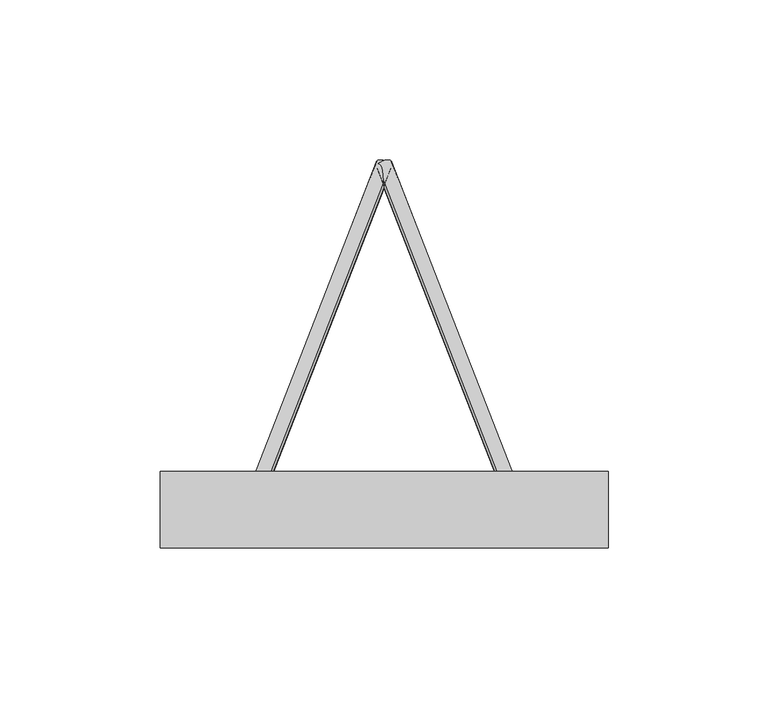
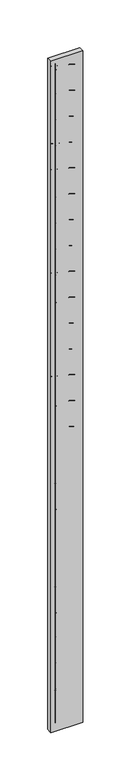
"""IFC4 building model written with IfcOpenShell, lengths in millimetres: proxy geometry, Vigota 1 (Pano 3) (Mf = 803)."""

from ifc_helpers import new_model, si_unit, point, frame, frame_2d, origin, origin_with_axes, origin_2d, place, context, project, spatial, polyline, circle_curve, trimmed, segment, composite_curve, outline, extrude, source, transform, mapped, element, save


def structural_framing_3061a772(model_context):
    return source(origin(), model_context, "Body", "SweptSolid", [
        extrude(outline(polyline([(-70.0, 12.0), (70.0, 12.0), (70.0, -12.0), (-70.0, -12.0), (-70.0, 12.0)])), origin_with_axes(), (0.0, 0.0, 1.0), 3115.00107),
        extrude(outline(composite_curve([segment(trimmed(circle_curve(origin_2d(), 2.5), [point((2.5, 0.0))], [point((-2.5, 0.0))], False, "CARTESIAN"), True, "CONTINUOUS"), segment(trimmed(circle_curve(origin_2d(), 2.5), [point((-2.5, 0.0))], [point((2.5, 0.0))], False, "CARTESIAN"), True, "CONTINUOUS")], self_intersect=False)), frame((0.0, 108.0, 1317.500535), z_axis=(0.3218603428886276, -0.8276408817707567, 0.4598004898837537), x_axis=(0.8192319205108605, -3.936835275445103e-11, -0.5734623443750141)), (0.0, 0.0, 1.0), 130.491379),
        extrude(outline(composite_curve([segment(trimmed(circle_curve(origin_2d(), 2.5), [point((2.5, 0.0))], [point((-2.5, 0.0))], False, "CARTESIAN"), True, "CONTINUOUS"), segment(trimmed(circle_curve(origin_2d(), 2.5), [point((-2.5, 0.0))], [point((2.5, 0.0))], False, "CARTESIAN"), True, "CONTINUOUS")], self_intersect=False)), frame((42.0, 0.0, 1377.500535), z_axis=(-0.3218603428886276, 0.8276408817707567, 0.4598004898837537), x_axis=(0.8192319205108605, -3.936835275445103e-11, 0.5734623443750141)), (0.0, 0.0, 1.0), 130.491379),
        extrude(outline(composite_curve([segment(trimmed(circle_curve(origin_2d(), 2.5), [point((2.5, 0.0))], [point((-2.5, 0.0))], False, "CARTESIAN"), True, "CONTINUOUS"), segment(trimmed(circle_curve(origin_2d(), 2.5), [point((-2.5, 0.0))], [point((2.5, 0.0))], False, "CARTESIAN"), True, "CONTINUOUS")], self_intersect=False)), frame((0.0, 108.0, 1437.500535), z_axis=(0.3218603428886276, -0.8276408817707567, 0.4598004898837537), x_axis=(0.8192319205108605, -3.936835275445103e-11, -0.5734623443750141)), (0.0, 0.0, 1.0), 130.491379),
        extrude(outline(composite_curve([segment(trimmed(circle_curve(origin_2d(), 2.5), [point((2.5, 0.0))], [point((-2.5, 0.0))], False, "CARTESIAN"), True, "CONTINUOUS"), segment(trimmed(circle_curve(origin_2d(), 2.5), [point((-2.5, 0.0))], [point((2.5, 0.0))], False, "CARTESIAN"), True, "CONTINUOUS")], self_intersect=False)), frame((42.0, 0.0, 1497.500535), z_axis=(-0.3218603428886276, 0.8276408817707567, 0.4598004898837537), x_axis=(0.8192319205108605, -3.936835275445103e-11, 0.5734623443750141)), (0.0, 0.0, 1.0), 130.491379),
        extrude(outline(composite_curve([segment(trimmed(circle_curve(origin_2d(), 2.5), [point((2.5, 0.0))], [point((-2.5, 0.0))], False, "CARTESIAN"), True, "CONTINUOUS"), segment(trimmed(circle_curve(origin_2d(), 2.5), [point((-2.5, 0.0))], [point((2.5, 0.0))], False, "CARTESIAN"), True, "CONTINUOUS")], self_intersect=False)), frame((0.0, 108.0, 1557.500535), z_axis=(0.3218603428886276, -0.8276408817707567, 0.4598004898837537), x_axis=(0.8192319205108605, -3.936835275445103e-11, -0.5734623443750141)), (0.0, 0.0, 1.0), 130.491379),
        extrude(outline(composite_curve([segment(trimmed(circle_curve(origin_2d(), 2.5), [point((2.5, 0.0))], [point((-2.5, 0.0))], False, "CARTESIAN"), True, "CONTINUOUS"), segment(trimmed(circle_curve(origin_2d(), 2.5), [point((-2.5, 0.0))], [point((2.5, 0.0))], False, "CARTESIAN"), True, "CONTINUOUS")], self_intersect=False)), frame((42.0, 0.0, 1617.500535), z_axis=(-0.3218603428886276, 0.8276408817707567, 0.4598004898837537), x_axis=(0.8192319205108605, -3.936835275445103e-11, 0.5734623443750141)), (0.0, 0.0, 1.0), 130.491379),
        extrude(outline(composite_curve([segment(trimmed(circle_curve(origin_2d(), 2.5), [point((2.5, 0.0))], [point((-2.5, 0.0))], False, "CARTESIAN"), True, "CONTINUOUS"), segment(trimmed(circle_curve(origin_2d(), 2.5), [point((-2.5, 0.0))], [point((2.5, 0.0))], False, "CARTESIAN"), True, "CONTINUOUS")], self_intersect=False)), frame((0.0, 108.0, 1677.500535), z_axis=(0.3218603428886276, -0.8276408817707567, 0.4598004898837537), x_axis=(0.8192319205108605, -3.936835275445103e-11, -0.5734623443750141)), (0.0, 0.0, 1.0), 130.491379),
        extrude(outline(composite_curve([segment(trimmed(circle_curve(origin_2d(), 2.5), [point((2.5, 0.0))], [point((-2.5, 0.0))], False, "CARTESIAN"), True, "CONTINUOUS"), segment(trimmed(circle_curve(origin_2d(), 2.5), [point((-2.5, 0.0))], [point((2.5, 0.0))], False, "CARTESIAN"), True, "CONTINUOUS")], self_intersect=False)), frame((42.0, 0.0, 1737.500535), z_axis=(-0.3218603428886276, 0.8276408817707567, 0.4598004898837537), x_axis=(0.8192319205108605, -3.936835275445103e-11, 0.5734623443750141)), (0.0, 0.0, 1.0), 130.491379),
        extrude(outline(composite_curve([segment(trimmed(circle_curve(origin_2d(), 2.5), [point((2.5, 0.0))], [point((-2.5, 0.0))], False, "CARTESIAN"), True, "CONTINUOUS"), segment(trimmed(circle_curve(origin_2d(), 2.5), [point((-2.5, 0.0))], [point((2.5, 0.0))], False, "CARTESIAN"), True, "CONTINUOUS")], self_intersect=False)), frame((0.0, 108.0, 1797.500535), z_axis=(0.3218603428886276, -0.8276408817707567, 0.4598004898837537), x_axis=(0.8192319205108605, -3.936835275445103e-11, -0.5734623443750141)), (0.0, 0.0, 1.0), 130.491379),
        extrude(outline(composite_curve([segment(trimmed(circle_curve(origin_2d(), 2.5), [point((2.5, 0.0))], [point((-2.5, 0.0))], False, "CARTESIAN"), True, "CONTINUOUS"), segment(trimmed(circle_curve(origin_2d(), 2.5), [point((-2.5, 0.0))], [point((2.5, 0.0))], False, "CARTESIAN"), True, "CONTINUOUS")], self_intersect=False)), frame((42.0, 0.0, 1857.500535), z_axis=(-0.3218603428886276, 0.8276408817707567, 0.4598004898837537), x_axis=(0.8192319205108605, -3.936835275445103e-11, 0.5734623443750141)), (0.0, 0.0, 1.0), 130.491379),
        extrude(outline(composite_curve([segment(trimmed(circle_curve(origin_2d(), 2.5), [point((2.5, 0.0))], [point((-2.5, 0.0))], False, "CARTESIAN"), True, "CONTINUOUS"), segment(trimmed(circle_curve(origin_2d(), 2.5), [point((-2.5, 0.0))], [point((2.5, 0.0))], False, "CARTESIAN"), True, "CONTINUOUS")], self_intersect=False)), frame((0.0, 108.0, 1917.500535), z_axis=(0.3218603428886276, -0.8276408817707567, 0.4598004898837537), x_axis=(0.8192319205108605, -3.936835275445103e-11, -0.5734623443750141)), (0.0, 0.0, 1.0), 130.491379),
        extrude(outline(composite_curve([segment(trimmed(circle_curve(origin_2d(), 2.5), [point((2.5, 0.0))], [point((-2.5, 0.0))], False, "CARTESIAN"), True, "CONTINUOUS"), segment(trimmed(circle_curve(origin_2d(), 2.5), [point((-2.5, 0.0))], [point((2.5, 0.0))], False, "CARTESIAN"), True, "CONTINUOUS")], self_intersect=False)), frame((42.0, 0.0, 1977.500535), z_axis=(-0.3218603428886276, 0.8276408817707567, 0.4598004898837537), x_axis=(0.8192319205108605, -3.936835275445103e-11, 0.5734623443750141)), (0.0, 0.0, 1.0), 130.491379),
        extrude(outline(composite_curve([segment(trimmed(circle_curve(origin_2d(), 2.5), [point((2.5, 0.0))], [point((-2.5, 0.0))], False, "CARTESIAN"), True, "CONTINUOUS"), segment(trimmed(circle_curve(origin_2d(), 2.5), [point((-2.5, 0.0))], [point((2.5, 0.0))], False, "CARTESIAN"), True, "CONTINUOUS")], self_intersect=False)), frame((0.0, 108.0, 2037.500535), z_axis=(0.3218603428886276, -0.8276408817707567, 0.4598004898837537), x_axis=(0.8192319205108605, -3.936835275445103e-11, -0.5734623443750141)), (0.0, 0.0, 1.0), 130.491379),
        extrude(outline(composite_curve([segment(trimmed(circle_curve(origin_2d(), 2.5), [point((2.5, 0.0))], [point((-2.5, 0.0))], False, "CARTESIAN"), True, "CONTINUOUS"), segment(trimmed(circle_curve(origin_2d(), 2.5), [point((-2.5, 0.0))], [point((2.5, 0.0))], False, "CARTESIAN"), True, "CONTINUOUS")], self_intersect=False)), frame((42.0, 0.0, 2097.500535), z_axis=(-0.3218603428886276, 0.8276408817707567, 0.4598004898837537), x_axis=(0.8192319205108605, -3.936835275445103e-11, 0.5734623443750141)), (0.0, 0.0, 1.0), 130.491379),
        extrude(outline(composite_curve([segment(trimmed(circle_curve(origin_2d(), 2.5), [point((2.5, 0.0))], [point((-2.5, 0.0))], False, "CARTESIAN"), True, "CONTINUOUS"), segment(trimmed(circle_curve(origin_2d(), 2.5), [point((-2.5, 0.0))], [point((2.5, 0.0))], False, "CARTESIAN"), True, "CONTINUOUS")], self_intersect=False)), frame((0.0, 108.0, 2157.500535), z_axis=(0.3218603428886276, -0.8276408817707567, 0.4598004898837537), x_axis=(0.8192319205108605, -3.936835275445103e-11, -0.5734623443750141)), (0.0, 0.0, 1.0), 130.491379),
        extrude(outline(composite_curve([segment(trimmed(circle_curve(origin_2d(), 2.5), [point((2.5, 0.0))], [point((-2.5, 0.0))], False, "CARTESIAN"), True, "CONTINUOUS"), segment(trimmed(circle_curve(origin_2d(), 2.5), [point((-2.5, 0.0))], [point((2.5, 0.0))], False, "CARTESIAN"), True, "CONTINUOUS")], self_intersect=False)), frame((42.0, 0.0, 2217.500535), z_axis=(-0.3218603428886276, 0.8276408817707567, 0.4598004898837537), x_axis=(0.8192319205108605, -3.936835275445103e-11, 0.5734623443750141)), (0.0, 0.0, 1.0), 130.491379),
        extrude(outline(composite_curve([segment(trimmed(circle_curve(origin_2d(), 2.5), [point((2.5, 0.0))], [point((-2.5, 0.0))], False, "CARTESIAN"), True, "CONTINUOUS"), segment(trimmed(circle_curve(origin_2d(), 2.5), [point((-2.5, 0.0))], [point((2.5, 0.0))], False, "CARTESIAN"), True, "CONTINUOUS")], self_intersect=False)), frame((0.0, 108.0, 2277.500535), z_axis=(0.3218603428886276, -0.8276408817707567, 0.4598004898837537), x_axis=(0.8192319205108605, -3.936835275445103e-11, -0.5734623443750141)), (0.0, 0.0, 1.0), 130.491379),
        extrude(outline(composite_curve([segment(trimmed(circle_curve(origin_2d(), 2.5), [point((2.5, 0.0))], [point((-2.5, 0.0))], False, "CARTESIAN"), True, "CONTINUOUS"), segment(trimmed(circle_curve(origin_2d(), 2.5), [point((-2.5, 0.0))], [point((2.5, 0.0))], False, "CARTESIAN"), True, "CONTINUOUS")], self_intersect=False)), frame((42.0, 0.0, 2337.500535), z_axis=(-0.3218603428886276, 0.8276408817707567, 0.4598004898837537), x_axis=(0.8192319205108605, -3.936835275445103e-11, 0.5734623443750141)), (0.0, 0.0, 1.0), 130.491379),
        extrude(outline(composite_curve([segment(trimmed(circle_curve(origin_2d(), 2.5), [point((2.5, 0.0))], [point((-2.5, 0.0))], False, "CARTESIAN"), True, "CONTINUOUS"), segment(trimmed(circle_curve(origin_2d(), 2.5), [point((-2.5, 0.0))], [point((2.5, 0.0))], False, "CARTESIAN"), True, "CONTINUOUS")], self_intersect=False)), frame((0.0, 108.0, 2397.500535), z_axis=(0.3218603428886276, -0.8276408817707567, 0.4598004898837537), x_axis=(0.8192319205108605, -3.936835275445103e-11, -0.5734623443750141)), (0.0, 0.0, 1.0), 130.491379),
        extrude(outline(composite_curve([segment(trimmed(circle_curve(origin_2d(), 2.5), [point((2.5, 0.0))], [point((-2.5, 0.0))], False, "CARTESIAN"), True, "CONTINUOUS"), segment(trimmed(circle_curve(origin_2d(), 2.5), [point((-2.5, 0.0))], [point((2.5, 0.0))], False, "CARTESIAN"), True, "CONTINUOUS")], self_intersect=False)), frame((42.0, 0.0, 2457.500535), z_axis=(-0.3218603428886276, 0.8276408817707567, 0.4598004898837537), x_axis=(0.8192319205108605, -3.936835275445103e-11, 0.5734623443750141)), (0.0, 0.0, 1.0), 130.491379),
        extrude(outline(composite_curve([segment(trimmed(circle_curve(origin_2d(), 2.5), [point((2.5, 0.0))], [point((-2.5, 0.0))], False, "CARTESIAN"), True, "CONTINUOUS"), segment(trimmed(circle_curve(origin_2d(), 2.5), [point((-2.5, 0.0))], [point((2.5, 0.0))], False, "CARTESIAN"), True, "CONTINUOUS")], self_intersect=False)), frame((0.0, 108.0, 2517.500535), z_axis=(0.3218603428886276, -0.8276408817707567, 0.4598004898837537), x_axis=(0.8192319205108605, -3.936835275445103e-11, -0.5734623443750141)), (0.0, 0.0, 1.0), 130.491379),
        extrude(outline(composite_curve([segment(trimmed(circle_curve(origin_2d(), 2.5), [point((2.5, 0.0))], [point((-2.5, 0.0))], False, "CARTESIAN"), True, "CONTINUOUS"), segment(trimmed(circle_curve(origin_2d(), 2.5), [point((-2.5, 0.0))], [point((2.5, 0.0))], False, "CARTESIAN"), True, "CONTINUOUS")], self_intersect=False)), frame((42.0, 0.0, 2577.500535), z_axis=(-0.3218603428886276, 0.8276408817707567, 0.4598004898837537), x_axis=(0.8192319205108605, -3.936835275445103e-11, 0.5734623443750141)), (0.0, 0.0, 1.0), 130.491379),
        extrude(outline(composite_curve([segment(trimmed(circle_curve(origin_2d(), 2.5), [point((2.5, 0.0))], [point((-2.5, 0.0))], False, "CARTESIAN"), True, "CONTINUOUS"), segment(trimmed(circle_curve(origin_2d(), 2.5), [point((-2.5, 0.0))], [point((2.5, 0.0))], False, "CARTESIAN"), True, "CONTINUOUS")], self_intersect=False)), frame((0.0, 108.0, 2637.500535), z_axis=(0.3218603428886276, -0.8276408817707567, 0.4598004898837537), x_axis=(0.8192319205108605, -3.936835275445103e-11, -0.5734623443750141)), (0.0, 0.0, 1.0), 130.491379),
        extrude(outline(composite_curve([segment(trimmed(circle_curve(origin_2d(), 2.5), [point((2.5, 0.0))], [point((-2.5, 0.0))], False, "CARTESIAN"), True, "CONTINUOUS"), segment(trimmed(circle_curve(origin_2d(), 2.5), [point((-2.5, 0.0))], [point((2.5, 0.0))], False, "CARTESIAN"), True, "CONTINUOUS")], self_intersect=False)), frame((42.0, 0.0, 2697.500535), z_axis=(-0.3218603428886276, 0.8276408817707567, 0.4598004898837537), x_axis=(0.8192319205108605, -3.936835275445103e-11, 0.5734623443750141)), (0.0, 0.0, 1.0), 130.491379),
        extrude(outline(composite_curve([segment(trimmed(circle_curve(origin_2d(), 2.5), [point((2.5, 0.0))], [point((-2.5, 0.0))], False, "CARTESIAN"), True, "CONTINUOUS"), segment(trimmed(circle_curve(origin_2d(), 2.5), [point((-2.5, 0.0))], [point((2.5, 0.0))], False, "CARTESIAN"), True, "CONTINUOUS")], self_intersect=False)), frame((0.0, 108.0, 2757.500535), z_axis=(0.3218603428886276, -0.8276408817707567, 0.4598004898837537), x_axis=(0.8192319205108605, -3.936835275445103e-11, -0.5734623443750141)), (0.0, 0.0, 1.0), 130.491379),
        extrude(outline(composite_curve([segment(trimmed(circle_curve(origin_2d(), 2.5), [point((2.5, 0.0))], [point((-2.5, 0.0))], False, "CARTESIAN"), True, "CONTINUOUS"), segment(trimmed(circle_curve(origin_2d(), 2.5), [point((-2.5, 0.0))], [point((2.5, 0.0))], False, "CARTESIAN"), True, "CONTINUOUS")], self_intersect=False)), frame((42.0, 0.0, 2817.500535), z_axis=(-0.3218603428886276, 0.8276408817707567, 0.4598004898837537), x_axis=(0.8192319205108605, -3.936835275445103e-11, 0.5734623443750141)), (0.0, 0.0, 1.0), 130.491379),
        extrude(outline(composite_curve([segment(trimmed(circle_curve(origin_2d(), 2.5), [point((2.5, 0.0))], [point((-2.5, 0.0))], False, "CARTESIAN"), True, "CONTINUOUS"), segment(trimmed(circle_curve(origin_2d(), 2.5), [point((-2.5, 0.0))], [point((2.5, 0.0))], False, "CARTESIAN"), True, "CONTINUOUS")], self_intersect=False)), frame((0.0, 108.0, 2877.500535), z_axis=(0.3218603428886276, -0.8276408817707567, 0.4598004898837537), x_axis=(0.8192319205108605, -3.936835275445103e-11, -0.5734623443750141)), (0.0, 0.0, 1.0), 130.491379),
        extrude(outline(composite_curve([segment(trimmed(circle_curve(origin_2d(), 2.5), [point((2.5, 0.0))], [point((-2.5, 0.0))], False, "CARTESIAN"), True, "CONTINUOUS"), segment(trimmed(circle_curve(origin_2d(), 2.5), [point((-2.5, 0.0))], [point((2.5, 0.0))], False, "CARTESIAN"), True, "CONTINUOUS")], self_intersect=False)), frame((42.0, 0.0, 2937.500535), z_axis=(-0.3218603428886276, 0.8276408817707567, 0.4598004898837537), x_axis=(0.8192319205108605, -3.936835275445103e-11, 0.5734623443750141)), (0.0, 0.0, 1.0), 130.491379),
        extrude(outline(composite_curve([segment(trimmed(circle_curve(origin_2d(), 2.5), [point((2.5, 0.0))], [point((-2.5, 0.0))], False, "CARTESIAN"), True, "CONTINUOUS"), segment(trimmed(circle_curve(origin_2d(), 2.5), [point((-2.5, 0.0))], [point((2.5, 0.0))], False, "CARTESIAN"), True, "CONTINUOUS")], self_intersect=False)), frame((0.0, 108.0, 2997.500535), z_axis=(0.3218603428886276, -0.8276408817707567, 0.4598004898837537), x_axis=(0.8192319205108605, -3.936835275445103e-11, -0.5734623443750141)), (0.0, 0.0, 1.0), 130.491379),
        extrude(outline(composite_curve([segment(trimmed(circle_curve(frame_2d((-42.0, 0.0)), 2.5), [point((-39.5, 0.0))], [point((-44.5, 0.0))], False, "CARTESIAN"), True, "CONTINUOUS"), segment(trimmed(circle_curve(frame_2d((-42.0, 0.0)), 2.5), [point((-44.5, 0.0))], [point((-39.5, 0.0))], False, "CARTESIAN"), True, "CONTINUOUS")], self_intersect=False)), frame((0.0, 0.0, 28.0), z_axis=(0.0, 0.0, 1.0), x_axis=(1.0, 0.0, 0.0)), (0.0, 0.0, 1.0), 3059.00107),
        extrude(outline(composite_curve([segment(trimmed(circle_curve(origin_2d(), 2.5), [point((2.5, 0.0))], [point((-2.5, 0.0))], False, "CARTESIAN"), True, "CONTINUOUS"), segment(trimmed(circle_curve(origin_2d(), 2.5), [point((-2.5, 0.0))], [point((2.5, 0.0))], False, "CARTESIAN"), True, "CONTINUOUS")], self_intersect=False)), frame((-42.0, 0.0, 57.500535), z_axis=(0.3218603428886276, 0.8276408817707567, 0.4598004898837537), x_axis=(0.8192319205108605, 3.936835275445103e-11, -0.5734623443750141)), (0.0, 0.0, 1.0), 130.491379),
        extrude(outline(composite_curve([segment(trimmed(circle_curve(origin_2d(), 2.5), [point((2.5, 0.0))], [point((-2.5, 0.0))], False, "CARTESIAN"), True, "CONTINUOUS"), segment(trimmed(circle_curve(origin_2d(), 2.5), [point((-2.5, 0.0))], [point((2.5, 0.0))], False, "CARTESIAN"), True, "CONTINUOUS")], self_intersect=False)), frame((0.0, 108.0, 117.500535), z_axis=(-0.3218603428886276, -0.8276408817707567, 0.4598004898837537), x_axis=(0.8192319205108605, 3.936835275445103e-11, 0.5734623443750141)), (0.0, 0.0, 1.0), 130.491379),
        extrude(outline(composite_curve([segment(trimmed(circle_curve(origin_2d(), 2.5), [point((2.5, 0.0))], [point((-2.5, 0.0))], False, "CARTESIAN"), True, "CONTINUOUS"), segment(trimmed(circle_curve(origin_2d(), 2.5), [point((-2.5, 0.0))], [point((2.5, 0.0))], False, "CARTESIAN"), True, "CONTINUOUS")], self_intersect=False)), frame((-42.0, 0.0, 177.500535), z_axis=(0.3218603428886276, 0.8276408817707567, 0.4598004898837537), x_axis=(0.8192319205108605, 3.936835275445103e-11, -0.5734623443750141)), (0.0, 0.0, 1.0), 130.491379),
        extrude(outline(composite_curve([segment(trimmed(circle_curve(origin_2d(), 2.5), [point((2.5, 0.0))], [point((-2.5, 0.0))], False, "CARTESIAN"), True, "CONTINUOUS"), segment(trimmed(circle_curve(origin_2d(), 2.5), [point((-2.5, 0.0))], [point((2.5, 0.0))], False, "CARTESIAN"), True, "CONTINUOUS")], self_intersect=False)), frame((0.0, 108.0, 237.500535), z_axis=(-0.3218603428886276, -0.8276408817707567, 0.4598004898837537), x_axis=(0.8192319205108605, 3.936835275445103e-11, 0.5734623443750141)), (0.0, 0.0, 1.0), 130.491379),
        extrude(outline(composite_curve([segment(trimmed(circle_curve(origin_2d(), 2.5), [point((2.5, 0.0))], [point((-2.5, 0.0))], False, "CARTESIAN"), True, "CONTINUOUS"), segment(trimmed(circle_curve(origin_2d(), 2.5), [point((-2.5, 0.0))], [point((2.5, 0.0))], False, "CARTESIAN"), True, "CONTINUOUS")], self_intersect=False)), frame((-42.0, 0.0, 297.500535), z_axis=(0.3218603428886276, 0.8276408817707567, 0.4598004898837537), x_axis=(0.8192319205108605, 3.936835275445103e-11, -0.5734623443750141)), (0.0, 0.0, 1.0), 130.491379),
        extrude(outline(composite_curve([segment(trimmed(circle_curve(origin_2d(), 2.5), [point((2.5, 0.0))], [point((-2.5, 0.0))], False, "CARTESIAN"), True, "CONTINUOUS"), segment(trimmed(circle_curve(origin_2d(), 2.5), [point((-2.5, 0.0))], [point((2.5, 0.0))], False, "CARTESIAN"), True, "CONTINUOUS")], self_intersect=False)), frame((0.0, 108.0, 357.500535), z_axis=(-0.3218603428886276, -0.8276408817707567, 0.4598004898837537), x_axis=(0.8192319205108605, 3.936835275445103e-11, 0.5734623443750141)), (0.0, 0.0, 1.0), 130.491379),
        extrude(outline(composite_curve([segment(trimmed(circle_curve(origin_2d(), 2.5), [point((2.5, 0.0))], [point((-2.5, 0.0))], False, "CARTESIAN"), True, "CONTINUOUS"), segment(trimmed(circle_curve(origin_2d(), 2.5), [point((-2.5, 0.0))], [point((2.5, 0.0))], False, "CARTESIAN"), True, "CONTINUOUS")], self_intersect=False)), frame((-42.0, 0.0, 417.500535), z_axis=(0.3218603428886276, 0.8276408817707567, 0.4598004898837537), x_axis=(0.8192319205108605, 3.936835275445103e-11, -0.5734623443750141)), (0.0, 0.0, 1.0), 130.491379),
        extrude(outline(composite_curve([segment(trimmed(circle_curve(origin_2d(), 2.5), [point((2.5, 0.0))], [point((-2.5, 0.0))], False, "CARTESIAN"), True, "CONTINUOUS"), segment(trimmed(circle_curve(origin_2d(), 2.5), [point((-2.5, 0.0))], [point((2.5, 0.0))], False, "CARTESIAN"), True, "CONTINUOUS")], self_intersect=False)), frame((0.0, 108.0, 477.500535), z_axis=(-0.3218603428886276, -0.8276408817707567, 0.4598004898837537), x_axis=(0.8192319205108605, 3.936835275445103e-11, 0.5734623443750141)), (0.0, 0.0, 1.0), 130.491379),
        extrude(outline(composite_curve([segment(trimmed(circle_curve(origin_2d(), 2.5), [point((2.5, 0.0))], [point((-2.5, 0.0))], False, "CARTESIAN"), True, "CONTINUOUS"), segment(trimmed(circle_curve(origin_2d(), 2.5), [point((-2.5, 0.0))], [point((2.5, 0.0))], False, "CARTESIAN"), True, "CONTINUOUS")], self_intersect=False)), frame((-42.0, 0.0, 537.500535), z_axis=(0.3218603428886276, 0.8276408817707567, 0.4598004898837537), x_axis=(0.8192319205108605, 3.936835275445103e-11, -0.5734623443750141)), (0.0, 0.0, 1.0), 130.491379),
        extrude(outline(composite_curve([segment(trimmed(circle_curve(origin_2d(), 2.5), [point((2.5, 0.0))], [point((-2.5, 0.0))], False, "CARTESIAN"), True, "CONTINUOUS"), segment(trimmed(circle_curve(origin_2d(), 2.5), [point((-2.5, 0.0))], [point((2.5, 0.0))], False, "CARTESIAN"), True, "CONTINUOUS")], self_intersect=False)), frame((0.0, 108.0, 597.500535), z_axis=(-0.3218603428886276, -0.8276408817707567, 0.4598004898837537), x_axis=(0.8192319205108605, 3.936835275445103e-11, 0.5734623443750141)), (0.0, 0.0, 1.0), 130.491379),
        extrude(outline(composite_curve([segment(trimmed(circle_curve(origin_2d(), 2.5), [point((2.5, 0.0))], [point((-2.5, 0.0))], False, "CARTESIAN"), True, "CONTINUOUS"), segment(trimmed(circle_curve(origin_2d(), 2.5), [point((-2.5, 0.0))], [point((2.5, 0.0))], False, "CARTESIAN"), True, "CONTINUOUS")], self_intersect=False)), frame((-42.0, 0.0, 657.500535), z_axis=(0.3218603428886276, 0.8276408817707567, 0.4598004898837537), x_axis=(0.8192319205108605, 3.936835275445103e-11, -0.5734623443750141)), (0.0, 0.0, 1.0), 130.491379),
        extrude(outline(composite_curve([segment(trimmed(circle_curve(origin_2d(), 2.5), [point((2.5, 0.0))], [point((-2.5, 0.0))], False, "CARTESIAN"), True, "CONTINUOUS"), segment(trimmed(circle_curve(origin_2d(), 2.5), [point((-2.5, 0.0))], [point((2.5, 0.0))], False, "CARTESIAN"), True, "CONTINUOUS")], self_intersect=False)), frame((0.0, 108.0, 717.500535), z_axis=(-0.3218603428886276, -0.8276408817707567, 0.4598004898837537), x_axis=(0.8192319205108605, 3.936835275445103e-11, 0.5734623443750141)), (0.0, 0.0, 1.0), 130.491379),
        extrude(outline(composite_curve([segment(trimmed(circle_curve(origin_2d(), 2.5), [point((2.5, 0.0))], [point((-2.5, 0.0))], False, "CARTESIAN"), True, "CONTINUOUS"), segment(trimmed(circle_curve(origin_2d(), 2.5), [point((-2.5, 0.0))], [point((2.5, 0.0))], False, "CARTESIAN"), True, "CONTINUOUS")], self_intersect=False)), frame((-42.0, 0.0, 777.500535), z_axis=(0.3218603428886276, 0.8276408817707567, 0.4598004898837537), x_axis=(0.8192319205108605, 3.936835275445103e-11, -0.5734623443750141)), (0.0, 0.0, 1.0), 130.491379),
        extrude(outline(composite_curve([segment(trimmed(circle_curve(origin_2d(), 2.5), [point((2.5, 0.0))], [point((-2.5, 0.0))], False, "CARTESIAN"), True, "CONTINUOUS"), segment(trimmed(circle_curve(origin_2d(), 2.5), [point((-2.5, 0.0))], [point((2.5, 0.0))], False, "CARTESIAN"), True, "CONTINUOUS")], self_intersect=False)), frame((0.0, 108.0, 837.500535), z_axis=(-0.3218603428886276, -0.8276408817707567, 0.4598004898837537), x_axis=(0.8192319205108605, 3.936835275445103e-11, 0.5734623443750141)), (0.0, 0.0, 1.0), 130.491379),
        extrude(outline(composite_curve([segment(trimmed(circle_curve(origin_2d(), 2.5), [point((2.5, 0.0))], [point((-2.5, 0.0))], False, "CARTESIAN"), True, "CONTINUOUS"), segment(trimmed(circle_curve(origin_2d(), 2.5), [point((-2.5, 0.0))], [point((2.5, 0.0))], False, "CARTESIAN"), True, "CONTINUOUS")], self_intersect=False)), frame((-42.0, 0.0, 897.500535), z_axis=(0.3218603428886276, 0.8276408817707567, 0.4598004898837537), x_axis=(0.8192319205108605, 3.936835275445103e-11, -0.5734623443750141)), (0.0, 0.0, 1.0), 130.491379),
        extrude(outline(composite_curve([segment(trimmed(circle_curve(origin_2d(), 2.5), [point((2.5, 0.0))], [point((-2.5, 0.0))], False, "CARTESIAN"), True, "CONTINUOUS"), segment(trimmed(circle_curve(origin_2d(), 2.5), [point((-2.5, 0.0))], [point((2.5, 0.0))], False, "CARTESIAN"), True, "CONTINUOUS")], self_intersect=False)), frame((0.0, 108.0, 957.500535), z_axis=(-0.3218603428886276, -0.8276408817707567, 0.4598004898837537), x_axis=(0.8192319205108605, 3.936835275445103e-11, 0.5734623443750141)), (0.0, 0.0, 1.0), 130.491379),
        extrude(outline(composite_curve([segment(trimmed(circle_curve(origin_2d(), 2.5), [point((2.5, 0.0))], [point((-2.5, 0.0))], False, "CARTESIAN"), True, "CONTINUOUS"), segment(trimmed(circle_curve(origin_2d(), 2.5), [point((-2.5, 0.0))], [point((2.5, 0.0))], False, "CARTESIAN"), True, "CONTINUOUS")], self_intersect=False)), frame((-42.0, 0.0, 1017.500535), z_axis=(0.3218603428886276, 0.8276408817707567, 0.4598004898837537), x_axis=(0.8192319205108605, 3.936835275445103e-11, -0.5734623443750141)), (0.0, 0.0, 1.0), 130.491379),
        extrude(outline(composite_curve([segment(trimmed(circle_curve(origin_2d(), 2.5), [point((2.5, 0.0))], [point((-2.5, 0.0))], False, "CARTESIAN"), True, "CONTINUOUS"), segment(trimmed(circle_curve(origin_2d(), 2.5), [point((-2.5, 0.0))], [point((2.5, 0.0))], False, "CARTESIAN"), True, "CONTINUOUS")], self_intersect=False)), frame((0.0, 108.0, 1077.500535), z_axis=(-0.3218603428886276, -0.8276408817707567, 0.4598004898837537), x_axis=(0.8192319205108605, 3.936835275445103e-11, 0.5734623443750141)), (0.0, 0.0, 1.0), 130.491379),
        extrude(outline(composite_curve([segment(trimmed(circle_curve(origin_2d(), 2.5), [point((2.5, 0.0))], [point((-2.5, 0.0))], False, "CARTESIAN"), True, "CONTINUOUS"), segment(trimmed(circle_curve(origin_2d(), 2.5), [point((-2.5, 0.0))], [point((2.5, 0.0))], False, "CARTESIAN"), True, "CONTINUOUS")], self_intersect=False)), frame((-42.0, 0.0, 1137.500535), z_axis=(0.3218603428886276, 0.8276408817707567, 0.4598004898837537), x_axis=(0.8192319205108605, 3.936835275445103e-11, -0.5734623443750141)), (0.0, 0.0, 1.0), 130.491379),
        extrude(outline(composite_curve([segment(trimmed(circle_curve(origin_2d(), 2.5), [point((2.5, 0.0))], [point((-2.5, 0.0))], False, "CARTESIAN"), True, "CONTINUOUS"), segment(trimmed(circle_curve(origin_2d(), 2.5), [point((-2.5, 0.0))], [point((2.5, 0.0))], False, "CARTESIAN"), True, "CONTINUOUS")], self_intersect=False)), frame((0.0, 108.0, 1197.500535), z_axis=(-0.3218603428886276, -0.8276408817707567, 0.4598004898837537), x_axis=(0.8192319205108605, 3.936835275445103e-11, 0.5734623443750141)), (0.0, 0.0, 1.0), 130.491379),
        extrude(outline(composite_curve([segment(trimmed(circle_curve(origin_2d(), 2.5), [point((2.5, 0.0))], [point((-2.5, 0.0))], False, "CARTESIAN"), True, "CONTINUOUS"), segment(trimmed(circle_curve(origin_2d(), 2.5), [point((-2.5, 0.0))], [point((2.5, 0.0))], False, "CARTESIAN"), True, "CONTINUOUS")], self_intersect=False)), frame((-42.0, 0.0, 1257.500535), z_axis=(0.3218603428886276, 0.8276408817707567, 0.4598004898837537), x_axis=(0.8192319205108605, 3.936835275445103e-11, -0.5734623443750141)), (0.0, 0.0, 1.0), 130.491379),
        extrude(outline(composite_curve([segment(trimmed(circle_curve(origin_2d(), 2.5), [point((2.5, 0.0))], [point((-2.5, 0.0))], False, "CARTESIAN"), True, "CONTINUOUS"), segment(trimmed(circle_curve(origin_2d(), 2.5), [point((-2.5, 0.0))], [point((2.5, 0.0))], False, "CARTESIAN"), True, "CONTINUOUS")], self_intersect=False)), frame((0.0, 108.0, 1317.500535), z_axis=(-0.3218603428886276, -0.8276408817707567, 0.4598004898837537), x_axis=(0.8192319205108605, 3.936835275445103e-11, 0.5734623443750141)), (0.0, 0.0, 1.0), 130.491379),
        extrude(outline(composite_curve([segment(trimmed(circle_curve(origin_2d(), 2.5), [point((2.5, 0.0))], [point((-2.5, 0.0))], False, "CARTESIAN"), True, "CONTINUOUS"), segment(trimmed(circle_curve(origin_2d(), 2.5), [point((-2.5, 0.0))], [point((2.5, 0.0))], False, "CARTESIAN"), True, "CONTINUOUS")], self_intersect=False)), frame((-42.0, 0.0, 1377.500535), z_axis=(0.3218603428886276, 0.8276408817707567, 0.4598004898837537), x_axis=(0.8192319205108605, 3.936835275445103e-11, -0.5734623443750141)), (0.0, 0.0, 1.0), 130.491379),
        extrude(outline(composite_curve([segment(trimmed(circle_curve(origin_2d(), 2.5), [point((2.5, 0.0))], [point((-2.5, 0.0))], False, "CARTESIAN"), True, "CONTINUOUS"), segment(trimmed(circle_curve(origin_2d(), 2.5), [point((-2.5, 0.0))], [point((2.5, 0.0))], False, "CARTESIAN"), True, "CONTINUOUS")], self_intersect=False)), frame((0.0, 108.0, 1437.500535), z_axis=(-0.3218603428886276, -0.8276408817707567, 0.4598004898837537), x_axis=(0.8192319205108605, 3.936835275445103e-11, 0.5734623443750141)), (0.0, 0.0, 1.0), 130.491379),
        extrude(outline(composite_curve([segment(trimmed(circle_curve(origin_2d(), 2.5), [point((2.5, 0.0))], [point((-2.5, 0.0))], False, "CARTESIAN"), True, "CONTINUOUS"), segment(trimmed(circle_curve(origin_2d(), 2.5), [point((-2.5, 0.0))], [point((2.5, 0.0))], False, "CARTESIAN"), True, "CONTINUOUS")], self_intersect=False)), frame((-42.0, 0.0, 1497.500535), z_axis=(0.3218603428886276, 0.8276408817707567, 0.4598004898837537), x_axis=(0.8192319205108605, 3.936835275445103e-11, -0.5734623443750141)), (0.0, 0.0, 1.0), 130.491379),
        extrude(outline(composite_curve([segment(trimmed(circle_curve(origin_2d(), 2.5), [point((2.5, 0.0))], [point((-2.5, 0.0))], False, "CARTESIAN"), True, "CONTINUOUS"), segment(trimmed(circle_curve(origin_2d(), 2.5), [point((-2.5, 0.0))], [point((2.5, 0.0))], False, "CARTESIAN"), True, "CONTINUOUS")], self_intersect=False)), frame((0.0, 108.0, 1557.500535), z_axis=(-0.3218603428886276, -0.8276408817707567, 0.4598004898837537), x_axis=(0.8192319205108605, 3.936835275445103e-11, 0.5734623443750141)), (0.0, 0.0, 1.0), 130.491379),
        extrude(outline(composite_curve([segment(trimmed(circle_curve(origin_2d(), 2.5), [point((2.5, 0.0))], [point((-2.5, 0.0))], False, "CARTESIAN"), True, "CONTINUOUS"), segment(trimmed(circle_curve(origin_2d(), 2.5), [point((-2.5, 0.0))], [point((2.5, 0.0))], False, "CARTESIAN"), True, "CONTINUOUS")], self_intersect=False)), frame((-42.0, 0.0, 1617.500535), z_axis=(0.3218603428886276, 0.8276408817707567, 0.4598004898837537), x_axis=(0.8192319205108605, 3.936835275445103e-11, -0.5734623443750141)), (0.0, 0.0, 1.0), 130.491379),
        extrude(outline(composite_curve([segment(trimmed(circle_curve(origin_2d(), 2.5), [point((2.5, 0.0))], [point((-2.5, 0.0))], False, "CARTESIAN"), True, "CONTINUOUS"), segment(trimmed(circle_curve(origin_2d(), 2.5), [point((-2.5, 0.0))], [point((2.5, 0.0))], False, "CARTESIAN"), True, "CONTINUOUS")], self_intersect=False)), frame((0.0, 108.0, 1677.500535), z_axis=(-0.3218603428886276, -0.8276408817707567, 0.4598004898837537), x_axis=(0.8192319205108605, 3.936835275445103e-11, 0.5734623443750141)), (0.0, 0.0, 1.0), 130.491379),
        extrude(outline(composite_curve([segment(trimmed(circle_curve(origin_2d(), 2.5), [point((2.5, 0.0))], [point((-2.5, 0.0))], False, "CARTESIAN"), True, "CONTINUOUS"), segment(trimmed(circle_curve(origin_2d(), 2.5), [point((-2.5, 0.0))], [point((2.5, 0.0))], False, "CARTESIAN"), True, "CONTINUOUS")], self_intersect=False)), frame((-42.0, 0.0, 1737.500535), z_axis=(0.3218603428886276, 0.8276408817707567, 0.4598004898837537), x_axis=(0.8192319205108605, 3.936835275445103e-11, -0.5734623443750141)), (0.0, 0.0, 1.0), 130.491379),
        extrude(outline(composite_curve([segment(trimmed(circle_curve(origin_2d(), 2.5), [point((2.5, 0.0))], [point((-2.5, 0.0))], False, "CARTESIAN"), True, "CONTINUOUS"), segment(trimmed(circle_curve(origin_2d(), 2.5), [point((-2.5, 0.0))], [point((2.5, 0.0))], False, "CARTESIAN"), True, "CONTINUOUS")], self_intersect=False)), frame((0.0, 108.0, 1797.500535), z_axis=(-0.3218603428886276, -0.8276408817707567, 0.4598004898837537), x_axis=(0.8192319205108605, 3.936835275445103e-11, 0.5734623443750141)), (0.0, 0.0, 1.0), 130.491379),
        extrude(outline(composite_curve([segment(trimmed(circle_curve(origin_2d(), 2.5), [point((2.5, 0.0))], [point((-2.5, 0.0))], False, "CARTESIAN"), True, "CONTINUOUS"), segment(trimmed(circle_curve(origin_2d(), 2.5), [point((-2.5, 0.0))], [point((2.5, 0.0))], False, "CARTESIAN"), True, "CONTINUOUS")], self_intersect=False)), frame((-42.0, 0.0, 1857.500535), z_axis=(0.3218603428886276, 0.8276408817707567, 0.4598004898837537), x_axis=(0.8192319205108605, 3.936835275445103e-11, -0.5734623443750141)), (0.0, 0.0, 1.0), 130.491379),
        extrude(outline(composite_curve([segment(trimmed(circle_curve(origin_2d(), 2.5), [point((2.5, 0.0))], [point((-2.5, 0.0))], False, "CARTESIAN"), True, "CONTINUOUS"), segment(trimmed(circle_curve(origin_2d(), 2.5), [point((-2.5, 0.0))], [point((2.5, 0.0))], False, "CARTESIAN"), True, "CONTINUOUS")], self_intersect=False)), frame((0.0, 108.0, 1917.500535), z_axis=(-0.3218603428886276, -0.8276408817707567, 0.4598004898837537), x_axis=(0.8192319205108605, 3.936835275445103e-11, 0.5734623443750141)), (0.0, 0.0, 1.0), 130.491379),
        extrude(outline(composite_curve([segment(trimmed(circle_curve(origin_2d(), 2.5), [point((2.5, 0.0))], [point((-2.5, 0.0))], False, "CARTESIAN"), True, "CONTINUOUS"), segment(trimmed(circle_curve(origin_2d(), 2.5), [point((-2.5, 0.0))], [point((2.5, 0.0))], False, "CARTESIAN"), True, "CONTINUOUS")], self_intersect=False)), frame((-42.0, 0.0, 1977.500535), z_axis=(0.3218603428886276, 0.8276408817707567, 0.4598004898837537), x_axis=(0.8192319205108605, 3.936835275445103e-11, -0.5734623443750141)), (0.0, 0.0, 1.0), 130.491379),
        extrude(outline(composite_curve([segment(trimmed(circle_curve(origin_2d(), 2.5), [point((2.5, 0.0))], [point((-2.5, 0.0))], False, "CARTESIAN"), True, "CONTINUOUS"), segment(trimmed(circle_curve(origin_2d(), 2.5), [point((-2.5, 0.0))], [point((2.5, 0.0))], False, "CARTESIAN"), True, "CONTINUOUS")], self_intersect=False)), frame((0.0, 108.0, 2037.500535), z_axis=(-0.3218603428886276, -0.8276408817707567, 0.4598004898837537), x_axis=(0.8192319205108605, 3.936835275445103e-11, 0.5734623443750141)), (0.0, 0.0, 1.0), 130.491379),
        extrude(outline(composite_curve([segment(trimmed(circle_curve(origin_2d(), 2.5), [point((2.5, 0.0))], [point((-2.5, 0.0))], False, "CARTESIAN"), True, "CONTINUOUS"), segment(trimmed(circle_curve(origin_2d(), 2.5), [point((-2.5, 0.0))], [point((2.5, 0.0))], False, "CARTESIAN"), True, "CONTINUOUS")], self_intersect=False)), frame((-42.0, 0.0, 2097.500535), z_axis=(0.3218603428886276, 0.8276408817707567, 0.4598004898837537), x_axis=(0.8192319205108605, 3.936835275445103e-11, -0.5734623443750141)), (0.0, 0.0, 1.0), 130.491379),
        extrude(outline(composite_curve([segment(trimmed(circle_curve(origin_2d(), 2.5), [point((2.5, 0.0))], [point((-2.5, 0.0))], False, "CARTESIAN"), True, "CONTINUOUS"), segment(trimmed(circle_curve(origin_2d(), 2.5), [point((-2.5, 0.0))], [point((2.5, 0.0))], False, "CARTESIAN"), True, "CONTINUOUS")], self_intersect=False)), frame((0.0, 108.0, 2157.500535), z_axis=(-0.3218603428886276, -0.8276408817707567, 0.4598004898837537), x_axis=(0.8192319205108605, 3.936835275445103e-11, 0.5734623443750141)), (0.0, 0.0, 1.0), 130.491379),
        extrude(outline(composite_curve([segment(trimmed(circle_curve(origin_2d(), 2.5), [point((2.5, 0.0))], [point((-2.5, 0.0))], False, "CARTESIAN"), True, "CONTINUOUS"), segment(trimmed(circle_curve(origin_2d(), 2.5), [point((-2.5, 0.0))], [point((2.5, 0.0))], False, "CARTESIAN"), True, "CONTINUOUS")], self_intersect=False)), frame((-42.0, 0.0, 2217.500535), z_axis=(0.3218603428886276, 0.8276408817707567, 0.4598004898837537), x_axis=(0.8192319205108605, 3.936835275445103e-11, -0.5734623443750141)), (0.0, 0.0, 1.0), 130.491379),
        extrude(outline(composite_curve([segment(trimmed(circle_curve(origin_2d(), 2.5), [point((2.5, 0.0))], [point((-2.5, 0.0))], False, "CARTESIAN"), True, "CONTINUOUS"), segment(trimmed(circle_curve(origin_2d(), 2.5), [point((-2.5, 0.0))], [point((2.5, 0.0))], False, "CARTESIAN"), True, "CONTINUOUS")], self_intersect=False)), frame((0.0, 108.0, 2277.500535), z_axis=(-0.3218603428886276, -0.8276408817707567, 0.4598004898837537), x_axis=(0.8192319205108605, 3.936835275445103e-11, 0.5734623443750141)), (0.0, 0.0, 1.0), 130.491379),
        extrude(outline(composite_curve([segment(trimmed(circle_curve(origin_2d(), 2.5), [point((2.5, 0.0))], [point((-2.5, 0.0))], False, "CARTESIAN"), True, "CONTINUOUS"), segment(trimmed(circle_curve(origin_2d(), 2.5), [point((-2.5, 0.0))], [point((2.5, 0.0))], False, "CARTESIAN"), True, "CONTINUOUS")], self_intersect=False)), frame((-42.0, 0.0, 2337.500535), z_axis=(0.3218603428886276, 0.8276408817707567, 0.4598004898837537), x_axis=(0.8192319205108605, 3.936835275445103e-11, -0.5734623443750141)), (0.0, 0.0, 1.0), 130.491379),
        extrude(outline(composite_curve([segment(trimmed(circle_curve(origin_2d(), 2.5), [point((2.5, 0.0))], [point((-2.5, 0.0))], False, "CARTESIAN"), True, "CONTINUOUS"), segment(trimmed(circle_curve(origin_2d(), 2.5), [point((-2.5, 0.0))], [point((2.5, 0.0))], False, "CARTESIAN"), True, "CONTINUOUS")], self_intersect=False)), frame((0.0, 108.0, 2397.500535), z_axis=(-0.3218603428886276, -0.8276408817707567, 0.4598004898837537), x_axis=(0.8192319205108605, 3.936835275445103e-11, 0.5734623443750141)), (0.0, 0.0, 1.0), 130.491379),
        extrude(outline(composite_curve([segment(trimmed(circle_curve(origin_2d(), 2.5), [point((2.5, 0.0))], [point((-2.5, 0.0))], False, "CARTESIAN"), True, "CONTINUOUS"), segment(trimmed(circle_curve(origin_2d(), 2.5), [point((-2.5, 0.0))], [point((2.5, 0.0))], False, "CARTESIAN"), True, "CONTINUOUS")], self_intersect=False)), frame((-42.0, 0.0, 2457.500535), z_axis=(0.3218603428886276, 0.8276408817707567, 0.4598004898837537), x_axis=(0.8192319205108605, 3.936835275445103e-11, -0.5734623443750141)), (0.0, 0.0, 1.0), 130.491379),
        extrude(outline(composite_curve([segment(trimmed(circle_curve(origin_2d(), 2.5), [point((2.5, 0.0))], [point((-2.5, 0.0))], False, "CARTESIAN"), True, "CONTINUOUS"), segment(trimmed(circle_curve(origin_2d(), 2.5), [point((-2.5, 0.0))], [point((2.5, 0.0))], False, "CARTESIAN"), True, "CONTINUOUS")], self_intersect=False)), frame((0.0, 108.0, 2517.500535), z_axis=(-0.3218603428886276, -0.8276408817707567, 0.4598004898837537), x_axis=(0.8192319205108605, 3.936835275445103e-11, 0.5734623443750141)), (0.0, 0.0, 1.0), 130.491379),
        extrude(outline(composite_curve([segment(trimmed(circle_curve(origin_2d(), 2.5), [point((2.5, 0.0))], [point((-2.5, 0.0))], False, "CARTESIAN"), True, "CONTINUOUS"), segment(trimmed(circle_curve(origin_2d(), 2.5), [point((-2.5, 0.0))], [point((2.5, 0.0))], False, "CARTESIAN"), True, "CONTINUOUS")], self_intersect=False)), frame((-42.0, 0.0, 2577.500535), z_axis=(0.3218603428886276, 0.8276408817707567, 0.4598004898837537), x_axis=(0.8192319205108605, 3.936835275445103e-11, -0.5734623443750141)), (0.0, 0.0, 1.0), 130.491379),
        extrude(outline(composite_curve([segment(trimmed(circle_curve(origin_2d(), 2.5), [point((2.5, 0.0))], [point((-2.5, 0.0))], False, "CARTESIAN"), True, "CONTINUOUS"), segment(trimmed(circle_curve(origin_2d(), 2.5), [point((-2.5, 0.0))], [point((2.5, 0.0))], False, "CARTESIAN"), True, "CONTINUOUS")], self_intersect=False)), frame((0.0, 108.0, 2637.500535), z_axis=(-0.3218603428886276, -0.8276408817707567, 0.4598004898837537), x_axis=(0.8192319205108605, 3.936835275445103e-11, 0.5734623443750141)), (0.0, 0.0, 1.0), 130.491379),
        extrude(outline(composite_curve([segment(trimmed(circle_curve(origin_2d(), 2.5), [point((2.5, 0.0))], [point((-2.5, 0.0))], False, "CARTESIAN"), True, "CONTINUOUS"), segment(trimmed(circle_curve(origin_2d(), 2.5), [point((-2.5, 0.0))], [point((2.5, 0.0))], False, "CARTESIAN"), True, "CONTINUOUS")], self_intersect=False)), frame((-42.0, 0.0, 2697.500535), z_axis=(0.3218603428886276, 0.8276408817707567, 0.4598004898837537), x_axis=(0.8192319205108605, 3.936835275445103e-11, -0.5734623443750141)), (0.0, 0.0, 1.0), 130.491379),
        extrude(outline(composite_curve([segment(trimmed(circle_curve(origin_2d(), 2.5), [point((2.5, 0.0))], [point((-2.5, 0.0))], False, "CARTESIAN"), True, "CONTINUOUS"), segment(trimmed(circle_curve(origin_2d(), 2.5), [point((-2.5, 0.0))], [point((2.5, 0.0))], False, "CARTESIAN"), True, "CONTINUOUS")], self_intersect=False)), frame((0.0, 108.0, 2757.500535), z_axis=(-0.3218603428886276, -0.8276408817707567, 0.4598004898837537), x_axis=(0.8192319205108605, 3.936835275445103e-11, 0.5734623443750141)), (0.0, 0.0, 1.0), 130.491379),
        extrude(outline(composite_curve([segment(trimmed(circle_curve(origin_2d(), 2.5), [point((2.5, 0.0))], [point((-2.5, 0.0))], False, "CARTESIAN"), True, "CONTINUOUS"), segment(trimmed(circle_curve(origin_2d(), 2.5), [point((-2.5, 0.0))], [point((2.5, 0.0))], False, "CARTESIAN"), True, "CONTINUOUS")], self_intersect=False)), frame((-42.0, 0.0, 2817.500535), z_axis=(0.3218603428886276, 0.8276408817707567, 0.4598004898837537), x_axis=(0.8192319205108605, 3.936835275445103e-11, -0.5734623443750141)), (0.0, 0.0, 1.0), 130.491379),
        extrude(outline(composite_curve([segment(trimmed(circle_curve(origin_2d(), 2.5), [point((2.5, 0.0))], [point((-2.5, 0.0))], False, "CARTESIAN"), True, "CONTINUOUS"), segment(trimmed(circle_curve(origin_2d(), 2.5), [point((-2.5, 0.0))], [point((2.5, 0.0))], False, "CARTESIAN"), True, "CONTINUOUS")], self_intersect=False)), frame((0.0, 108.0, 2877.500535), z_axis=(-0.3218603428886276, -0.8276408817707567, 0.4598004898837537), x_axis=(0.8192319205108605, 3.936835275445103e-11, 0.5734623443750141)), (0.0, 0.0, 1.0), 130.491379),
        extrude(outline(composite_curve([segment(trimmed(circle_curve(origin_2d(), 2.5), [point((2.5, 0.0))], [point((-2.5, 0.0))], False, "CARTESIAN"), True, "CONTINUOUS"), segment(trimmed(circle_curve(origin_2d(), 2.5), [point((-2.5, 0.0))], [point((2.5, 0.0))], False, "CARTESIAN"), True, "CONTINUOUS")], self_intersect=False)), frame((-42.0, 0.0, 2937.500535), z_axis=(0.3218603428886276, 0.8276408817707567, 0.4598004898837537), x_axis=(0.8192319205108605, 3.936835275445103e-11, -0.5734623443750141)), (0.0, 0.0, 1.0), 130.491379),
        extrude(outline(composite_curve([segment(trimmed(circle_curve(origin_2d(), 2.5), [point((2.5, 0.0))], [point((-2.5, 0.0))], False, "CARTESIAN"), True, "CONTINUOUS"), segment(trimmed(circle_curve(origin_2d(), 2.5), [point((-2.5, 0.0))], [point((2.5, 0.0))], False, "CARTESIAN"), True, "CONTINUOUS")], self_intersect=False)), frame((0.0, 108.0, 2997.500535), z_axis=(-0.3218603428886276, -0.8276408817707567, 0.4598004898837537), x_axis=(0.8192319205108605, 3.936835275445103e-11, 0.5734623443750141)), (0.0, 0.0, 1.0), 130.491379),
        extrude(outline(composite_curve([segment(trimmed(circle_curve(frame_2d((42.0, 0.0)), 2.5), [point((44.5, 0.0))], [point((39.5, 0.0))], False, "CARTESIAN"), True, "CONTINUOUS"), segment(trimmed(circle_curve(frame_2d((42.0, 0.0)), 2.5), [point((39.5, 0.0))], [point((44.5, 0.0))], False, "CARTESIAN"), True, "CONTINUOUS")], self_intersect=False)), frame((0.0, 0.0, 28.0), z_axis=(0.0, 0.0, 1.0), x_axis=(1.0, 0.0, 0.0)), (0.0, 0.0, 1.0), 3059.00107),
    ])


if __name__ == "__main__":
    model = new_model("IFC4")
    model_context = context("Model", 3, world=origin())
    ifc_project = project(units=[si_unit("LENGTHUNIT", "METRE", prefix="MILLI")], contexts=[model_context])
    site = spatial("IfcSite", under=ifc_project)
    building = spatial("IfcBuilding", under=site)
    placement = place(None, origin())
    structural_framing_shape = structural_framing_3061a772(model_context)
    element("IfcBuildingElementProxy", 1, Name="Vigota 1 (Pano 3) (Mf = 803)", ObjectType="Vigota 1 (Pano 3) (Mf = 803)", at=placement, inside=building, context=model_context, shape_type="MappedRepresentation", body=[
        mapped(structural_framing_shape, transform((0.0, 0.0, 0.0), x_axis=(1.0, 0.0, 0.0), y_axis=(0.0, 1.0, 0.0), z_axis=(0.0, 0.0, 1.0))),
    ])
    save(model, "model.ifc")

# Revit data of these elements
# Element 1 (IfcBuildingElementProxy, "Vigota 1 (Pano 3) (Mf = 803)")
#   Materials on its faces: "Aço", "Concreto armado"
# Materials
#   "Aço": class "Metal", colour RGB 120 120 120, transparency 0, Description = "Aço estrutural A36 grau, ASTM B, acabamento laminado", Cost = 0
#   "Concreto armado": class "Não atribuído", colour RGB 168 169 158, transparency 0
